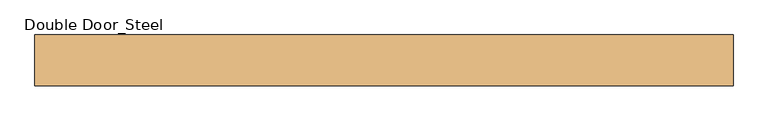
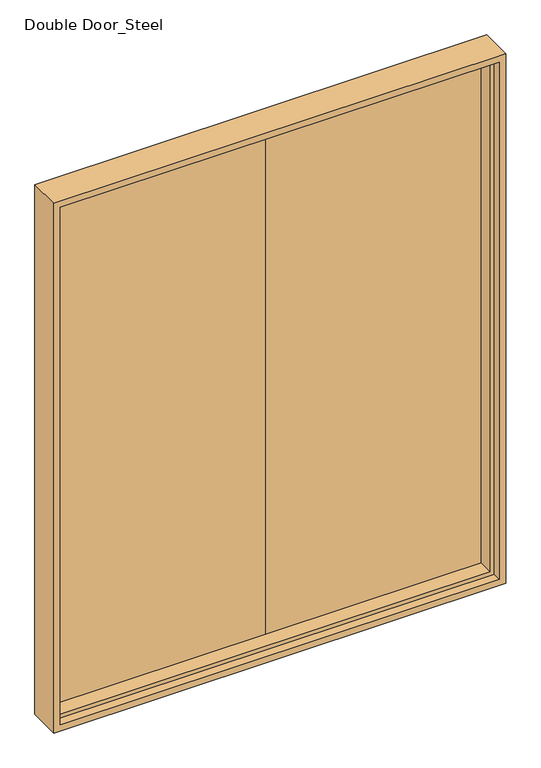
"""IFC4 building model written with IfcOpenShell, lengths in millimetres: door geometry, Double Door_Steel : H_DR_AR B12_Door_Double_W2100xH2580_FR 1.0H_FSD-5."""

import ifcopenshell
import ifcopenshell.guid

model = None  # the IFC model being written
_history = None  # IfcOwnerHistory: only IFC2X3 demands one
_inside = {}  # id of a spatial element -> (the spatial element, [elements in it])
_under = {}  # id of a project, library or spatial element -> (it, [spatial elements below it])
_declared = {}  # id of a project -> (the project, [libraries it declares])
_typed = {}  # id of a type object -> (the type object, [elements of that type])
_made_of = {}  # id of a material, layer set ... -> (it, [elements and type objects made of it])


def new_model(schema):
    """Start an empty IFC model of exactly this schema.

    Asked for "IFC4X3", IfcOpenShell would pick the latest addendum, in which some entities
    have other attributes; the version numbers below select the first issue.
    IFC2X3 requires an IfcOwnerHistory on every rooted entity: one is made here for all.
    """
    global model, _history
    if schema == "IFC4X3":
        model = ifcopenshell.file(schema_version=(4, 3, 0, 0))
    else:
        model = ifcopenshell.file(schema=schema)
    _inside.clear()
    _under.clear()
    _declared.clear()
    _typed.clear()
    _made_of.clear()
    _history = None
    if model.schema == "IFC2X3":
        org = make("IfcOrganization", Name="unknown")
        user = make(
            "IfcPersonAndOrganization",
            ThePerson=make("IfcPerson", FamilyName="unknown"),
            TheOrganization=org,
        )
        app = make(
            "IfcApplication",
            ApplicationDeveloper=org,
            Version="unknown",
            ApplicationFullName="unknown",
            ApplicationIdentifier="unknown",
        )
        _history = make(
            "IfcOwnerHistory",
            OwningUser=user,
            OwningApplication=app,
            ChangeAction="ADDED",
            CreationDate=0,
        )
    return model


def make(cls, **values):
    """One entity of the class cls with the attributes given. An attribute that is None is left unset."""
    return model.create_entity(
        cls, **{name: value for name, value in values.items() if value is not None}
    )


def rooted(cls, **values):
    """An entity with a GlobalId (a new one), such as an element, a storey or a relation."""
    return make(cls, GlobalId=ifcopenshell.guid.new(), OwnerHistory=_history, **values)


def si_unit(unit_type, name, prefix=None):
    """IfcSIUnit, for example si_unit("LENGTHUNIT", "METRE", prefix="MILLI")."""
    return make("IfcSIUnit", UnitType=unit_type, Prefix=prefix, Name=name)


def assignment(units):
    """IfcUnitAssignment: the units of a project."""
    return None if units is None else make("IfcUnitAssignment", Units=units)


def point(xyz):
    """IfcCartesianPoint."""
    return None if xyz is None else make("IfcCartesianPoint", Coordinates=xyz)


def direction(xyz):
    """IfcDirection."""
    return None if xyz is None else make("IfcDirection", DirectionRatios=xyz)


def frame(location, z_axis=None, x_axis=None):
    """IfcAxis2Placement3D, a coordinate frame: its origin and axes. An axis left out is left unset."""
    return make(
        "IfcAxis2Placement3D",
        Location=point(location),
        Axis=direction(z_axis),
        RefDirection=direction(x_axis),
    )


def origin():
    """The frame at (0, 0, 0) with its axes left unset."""
    return frame((0.0, 0.0, 0.0))


def place(relative_to, where):
    """IfcLocalPlacement: puts the frame where relative to a parent placement (None: the world)."""
    return make(
        "IfcLocalPlacement", PlacementRelTo=relative_to, RelativePlacement=where
    )


def context(
    kind, dimensions, precision=None, world=None, true_north=None, identifier=None
):
    """IfcGeometricRepresentationContext, for example the 3D "Model" context."""
    return make(
        "IfcGeometricRepresentationContext",
        ContextIdentifier=identifier,
        ContextType=kind,
        CoordinateSpaceDimension=dimensions,
        Precision=precision,
        WorldCoordinateSystem=world,
        TrueNorth=true_north,
    )


def project(units=None, contexts=None):
    """IfcProject with its units and contexts."""
    return rooted(
        "IfcProject",
        Name="project",
        RepresentationContexts=contexts,
        UnitsInContext=assignment(units),
    )


def spatial(cls, under=None, at=None, **own):
    """A site, building, storey or space (cls), placed at a placement, below another one or the project."""
    s = rooted(cls, ObjectPlacement=at, **own)
    if under is not None:
        _under.setdefault(under.id(), (under, []))[1].append(s)
    return s


def polyline(points):
    """IfcPolyline through the points."""
    return make("IfcPolyline", Points=[point(p) for p in points])


def outline(outer, holes=None, kind="AREA"):
    """IfcArbitraryClosedProfileDef: a profile drawn as a closed curve; with holes, ...WithVoids."""
    if holes is None:
        return make("IfcArbitraryClosedProfileDef", ProfileType=kind, OuterCurve=outer)
    return make(
        "IfcArbitraryProfileDefWithVoids",
        ProfileType=kind,
        OuterCurve=outer,
        InnerCurves=holes,
    )


def extrude(swept, where, along, depth):
    """IfcExtrudedAreaSolid: the profile swept, set in the frame where, extruded along a direction by depth."""
    return make(
        "IfcExtrudedAreaSolid",
        SweptArea=swept,
        Position=where,
        ExtrudedDirection=direction(along),
        Depth=depth,
    )


def faces_of(points, faces, orient=None, outer=None):
    """IfcFace entities. A face is a list of loops; a loop is a list of indices into points, from 0.

    orient and outer hold one flag for each loop. By default every Orientation is true, the
    first loop of a face is its IfcFaceOuterBound and the others are IfcFaceBound.
    """
    made = []
    for i, loops in enumerate(faces):
        bounds = []
        for j, loop in enumerate(loops):
            is_outer = j == 0 if outer is None else outer[i][j]
            bounds.append(
                make(
                    "IfcFaceOuterBound" if is_outer else "IfcFaceBound",
                    Bound=make("IfcPolyLoop", Polygon=[points[k] for k in loop]),
                    Orientation=True if orient is None else orient[i][j],
                )
            )
        made.append(make("IfcFace", Bounds=bounds))
    return made


def faceted_brep(points, faces, orient=None, outer=None, voids=None):
    """IfcFacetedBrep: a solid bounded by flat faces; with voids (closed shells), ...WithVoids."""
    shared = [point(p) for p in points]
    hull = make("IfcClosedShell", CfsFaces=faces_of(shared, faces, orient, outer))
    if voids is None:
        return make("IfcFacetedBrep", Outer=hull)
    return make(
        "IfcFacetedBrepWithVoids",
        Outer=hull,
        Voids=[
            make(cls, CfsFaces=faces_of(shared, fs, o, b)) for cls, fs, o, b in voids
        ],
    )


def shape(context_of_items, identifier, shape_type, items):
    """IfcShapeRepresentation: the items that make up one representation, for example the "Body"."""
    return make(
        "IfcShapeRepresentation",
        ContextOfItems=context_of_items,
        RepresentationIdentifier=identifier,
        RepresentationType=shape_type,
        Items=items,
    )


def source(mapping_origin, context_of_items, identifier, shape_type, items):
    """IfcRepresentationMap: a shape defined once, which mapped items show again and again."""
    return make(
        "IfcRepresentationMap",
        MappingOrigin=mapping_origin,
        MappedRepresentation=shape(context_of_items, identifier, shape_type, items),
    )


def transform(
    local_origin,
    x_axis=None,
    y_axis=None,
    z_axis=None,
    scale=None,
    scale2=None,
    scale3=None,
    uniform=True,
):
    """IfcCartesianTransformationOperator3D, or its non-uniform kind. x_axis, y_axis, z_axis: its Axis1, 2, 3."""
    if uniform:
        return make(
            "IfcCartesianTransformationOperator3D",
            Axis1=direction(x_axis),
            Axis2=direction(y_axis),
            LocalOrigin=point(local_origin),
            Scale=scale,
            Axis3=direction(z_axis),
        )
    return make(
        "IfcCartesianTransformationOperator3DnonUniform",
        Axis1=direction(x_axis),
        Axis2=direction(y_axis),
        LocalOrigin=point(local_origin),
        Scale=scale,
        Axis3=direction(z_axis),
        Scale2=scale2,
        Scale3=scale3,
    )


def mapped(mapping_source, mapping_target):
    """IfcMappedItem: shows the shape of a source again, moved by a transform."""
    return make(
        "IfcMappedItem", MappingSource=mapping_source, MappingTarget=mapping_target
    )


def made_of(thing, what):
    """Note that an element or type object is made of a material, layer set ...; save() writes the relation."""
    if what is not None:
        _made_of.setdefault(what.id(), (what, []))[1].append(thing)
    return thing


def element(
    cls,
    number,
    at=None,
    inside=None,
    cuts=None,
    type_object=None,
    material=None,
    context=None,
    identifier="Body",
    shape_type=None,
    held_by="IfcProductDefinitionShape",
    body=None,
    shapes=None,
    **own,
):
    """One element of the class cls, such as IfcWall. Its Tag is "e" and its number.

    at: its placement. inside: the storey or other place that contains it. cuts: it is an
    opening in that element (IfcRelVoidsElement). A single representation is given by context,
    identifier, shape_type and body (its items); several are given by shapes. held_by: the class
    of the entity that holds the representations. save() writes the other relations.
    """
    e = rooted(cls, Tag="e%d" % number, ObjectPlacement=at, **own)
    if body is not None:
        shapes = [shape(context, identifier, shape_type, body)]
    if shapes is not None:
        e.Representation = make(held_by, Representations=shapes)
    if inside is not None:
        _inside.setdefault(inside.id(), (inside, []))[1].append(e)
    if cuts is not None:
        rooted(
            "IfcRelVoidsElement", RelatingBuildingElement=cuts, RelatedOpeningElement=e
        )
    if type_object is not None:
        _typed.setdefault(type_object.id(), (type_object, []))[1].append(e)
    return made_of(e, material)


def aggregate(whole, parts):
    """IfcRelAggregates: a whole, such as a stair, and the parts it consists of."""
    return rooted("IfcRelAggregates", RelatingObject=whole, RelatedObjects=parts)


def save(model, path):
    """Write the relations noted so far, then the file.

    IfcRelAggregates (storeys below a building ...), IfcRelContainedInSpatialStructure (elements
    in a storey), IfcRelDefinesByType, IfcRelAssociatesMaterial and IfcRelDeclares: one each for
    every whole, place, type object, material and project.
    """
    for whole, parts in _under.values():
        aggregate(whole, parts)
    for where, things in _inside.values():
        rooted(
            "IfcRelContainedInSpatialStructure",
            RelatedElements=things,
            RelatingStructure=where,
        )
    for kind, things in _typed.values():
        rooted("IfcRelDefinesByType", RelatedObjects=things, RelatingType=kind)
    for what, things in _made_of.values():
        rooted("IfcRelAssociatesMaterial", RelatedObjects=things, RelatingMaterial=what)
    for by, libraries in _declared.values():
        rooted("IfcRelDeclares", RelatingContext=by, RelatedDefinitions=libraries)
    model.write(path)


def double_door_steel_b4304629(model_context):
    return source(origin(), model_context, "Body", "SolidModel", [
        faceted_brep([(-1035.0, -75.0, 2565.0), (-1035.0, 75.0, 2565.0), (-1035.0, 75.0, 0.0), (-1035.0, -75.0, 0.0), (1035.0, 75.0, 0.0), (1035.0, 75.0, 2565.0), (1005.0, 75.0, 2535.0), (-1005.0, 75.0, 2535.0), (-1005.0, 75.0, 30.0), (1005.0, 75.0, 30.0), (1035.0, -75.0, 0.0), (1035.0, -75.0, 2565.0), (1005.0, -75.0, 30.0), (-1005.0, -75.0, 30.0), (-1005.0, -75.0, 2535.0), (1005.0, -75.0, 2535.0), (-1005.0, -35.0, 2535.0), (-1005.0, -35.0, 30.0), (1005.0, -35.0, 30.0), (1005.0, -35.0, 2535.0), (985.0, -35.0, 2515.0), (985.0, -35.0, 50.0), (-985.0, -35.0, 50.0), (-985.0, -35.0, 2515.0), (-985.0, 35.0, 2515.0), (-985.0, 35.0, 50.0), (985.0, 35.0, 50.0), (1005.0, 35.0, 30.0), (-1005.0, 35.0, 30.0), (-1005.0, 35.0, 2535.0), (1005.0, 35.0, 2535.0), (985.0, 35.0, 2515.0)], [[[0, 1, 2, 3]], [[4, 2, 1, 5], [6, 7, 8, 9]], [[3, 2, 4, 10]], [[11, 0, 3, 10], [12, 13, 14, 15]], [[16, 14, 13, 17]], [[17, 13, 12, 18]], [[16, 17, 18, 19], [20, 21, 22, 23]], [[24, 23, 22, 25]], [[25, 22, 21, 26]], [[27, 28, 29, 30], [31, 24, 25, 26]], [[7, 29, 28, 8]], [[8, 28, 27, 9]], [[10, 4, 5, 11]], [[9, 27, 30, 6]], [[18, 12, 15, 19]], [[26, 21, 20, 31]], [[11, 5, 1, 0]], [[19, 15, 14, 16]], [[31, 20, 23, 24]], [[6, 30, 29, 7]]]),
        extrude(outline(polyline([(1005.0, 35.0), (0.0, 35.0), (0.0, 75.0), (1005.0, 75.0), (1005.0, 35.0)])), frame((0.0, 0.0, 30.0), z_axis=(0.0, 0.0, 1.0), x_axis=(1.0, 0.0, 0.0)), (0.0, 0.0, 1.0), 2505.0),
        extrude(outline(polyline([(0.0, 35.0), (-1005.0, 35.0), (-1005.0, 75.0), (0.0, 75.0), (0.0, 35.0)])), frame((0.0, 0.0, 30.0), z_axis=(0.0, 0.0, 1.0), x_axis=(1.0, 0.0, 0.0)), (0.0, 0.0, 1.0), 2505.0),
    ])


if __name__ == "__main__":
    model = new_model("IFC4")
    model_context = context("Model", 3, world=origin())
    ifc_project = project(units=[si_unit("LENGTHUNIT", "METRE", prefix="MILLI")], contexts=[model_context])
    site = spatial("IfcSite", under=ifc_project)
    building = spatial("IfcBuilding", under=site)
    placement = place(None, origin())
    double_door_steel_shape = double_door_steel_b4304629(model_context)
    element("IfcDoor", 1, ObjectType="Double Door_Steel : H_DR_AR B12_Door_Double_W2100xH2580_FR 1.0H_FSD-5", at=placement, inside=building, context=model_context, shape_type="MappedRepresentation", body=[
        mapped(double_door_steel_shape, transform((0.0, 0.0, 0.0), x_axis=(1.0, 0.0, 0.0), y_axis=(0.0, 1.0, 0.0), z_axis=(0.0, 0.0, 1.0))),
    ])
    save(model, "model.ifc")

# Revit data of these elements
# Type "Double Door_Steel : H_DR_AR B12_Door_Double_W2100xH2580_FR 1.0H_FSD-5"
#   Type Mark = "447"
#   프레임 = ""
#   철물 = ""
#   유리/마감 = ""
#   위치/개소 = ""
#   부호 = ""
#   문번호 = ""
#   문기호 = "FSD-4"
#   Analytic Construction = "<None>"
#   Door Width = 1005 mm
#   Height = 2580 mm
#   Width = 2100 mm
#   Define Thermal Properties by = 1
#   문 틀 = none
#   문 = none
#   Function = (empty or 0)
#   Assembly Code = ""
#   Wall Closure = (empty or 0)
